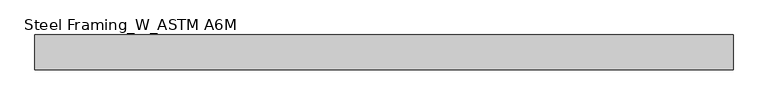
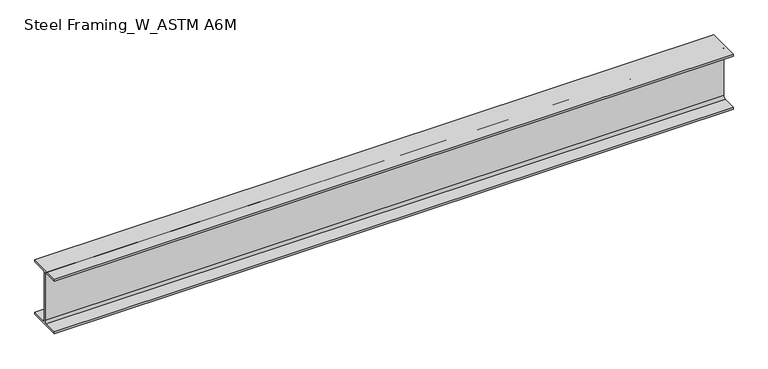
"""IFC4 building model written with IfcOpenShell, lengths in millimetres: beam geometry, Steel Framing_W_ASTM A6M : H_SB_ASB_W360x64."""

from ifc_helpers import new_model, si_unit, point, frame, frame_2d, origin, place, context, project, spatial, polyline, circle_curve, trimmed, segment, composite_curve, outline, extrude, source, transform, mapped, element, save


def steel_framing_w_astm_a6m_37d654f5(model_context):
    return source(origin(), model_context, "Body", "SweptSolid", [
        extrude(outline(composite_curve([segment(polyline([(101.5, -160.5), (101.5, -174.0), (-101.5, -174.0), (-101.5, -160.5), (-18.775, -160.5)]), True, "CONTINUOUS"), segment(trimmed(circle_curve(frame_2d((-18.775, -145.6)), 14.9), [point((-18.775, -160.5))], [point((-3.875, -145.6))], True, "CARTESIAN"), True, "CONTINUOUS"), segment(polyline([(-3.875, -145.6), (-3.875, 145.6)]), True, "CONTINUOUS"), segment(trimmed(circle_curve(frame_2d((-18.775, 145.6)), 14.9), [point((-3.875, 145.6))], [point((-18.775, 160.5))], True, "CARTESIAN"), True, "CONTINUOUS"), segment(polyline([(-18.775, 160.5), (-101.5, 160.5), (-101.5, 174.0), (101.5, 174.0), (101.5, 160.5), (18.775, 160.5)]), True, "CONTINUOUS"), segment(trimmed(circle_curve(frame_2d((18.775, 145.6)), 14.9), [point((18.775, 160.5))], [point((3.875, 145.6))], True, "CARTESIAN"), True, "CONTINUOUS"), segment(polyline([(3.875, 145.6), (3.875, -145.6)]), True, "CONTINUOUS"), segment(trimmed(circle_curve(frame_2d((18.775, -145.6)), 14.9), [point((3.875, -145.6))], [point((18.775, -160.5))], True, "CARTESIAN"), True, "CONTINUOUS"), segment(polyline([(18.775, -160.5), (101.5, -160.5)]), True, "CONTINUOUS")], self_intersect=False)), frame((-2037.3, 0.0, 0.0), z_axis=(1.0, 0.0, 0.0), x_axis=(0.0, 1.0, 0.0)), (0.0, 0.0, 1.0), 4074.6),
    ])


if __name__ == "__main__":
    model = new_model("IFC4")
    model_context = context("Model", 3, world=origin())
    ifc_project = project(units=[si_unit("LENGTHUNIT", "METRE", prefix="MILLI")], contexts=[model_context])
    site = spatial("IfcSite", under=ifc_project)
    building = spatial("IfcBuilding", under=site)
    placement = place(None, origin())
    steel_framing_w_astm_a6m_shape = steel_framing_w_astm_a6m_37d654f5(model_context)
    element("IfcBeam", 1, ObjectType="Steel Framing_W_ASTM A6M : H_SB_ASB_W360x64", at=placement, inside=building, context=model_context, shape_type="MappedRepresentation", body=[
        mapped(steel_framing_w_astm_a6m_shape, transform((0.0, 0.0, 0.0), x_axis=(1.0, 0.0, 0.0), y_axis=(0.0, 1.0, 0.0), z_axis=(0.0, 0.0, 1.0))),
    ])
    save(model, "model.ifc")

# Revit data of these elements
# Type "Steel Framing_W_ASTM A6M : H_SB_ASB_W360x64"
#   Section Name Key = "W14x43"
#   Width = 20.3 cm
#   Web Thickness = 0.775 cm
#   Web Fillet = 1.49 cm
#   Warping Constant = 524000.0 cm⁶
#   Torsional Moment of Inertia = 43.70 cm⁴
#   Section Area = 81.3 cm²
#   Plastic Modulus weak axis = 283.0 cm³
#   Plastic Modulus strong axis = 1140.0 cm³
#   Perimeter = 1.47 m²/m
#   Nominal Weight = 64.00 kgf/m
#   Moment of Inertia weak axis = 1880.00 cm⁴
#   Moment of Inertia strong axis = 17800.00 cm⁴
#   Height = 34.8 cm
#   Flange Thickness = 1.35 cm
#   Elastic Modulus weak axis = 185.0 cm³
#   Elastic Modulus strong axis = 1030.0 cm³
#   Centroid Vertical = 17.4 cm
#   Centroid Horizontal = 10.15 cm
#   Length [instance default] = 1500.000 mm
#   Structural Material [instance default] = Steel, 45-345
#   Bolt Spacing = 0
#   Assembly Code = ""
# Element 1 (IfcBeam, "Steel Framing_W_ASTM A6M : H_SB_ASB_W360x64")
#   Materials on its faces: "Steel, 45-345"
# Materials
#   "Steel, 45-345": class "Metal", colour RGB 189 187 185, transparency 0, Description = "Steel 345 MPa", Cost = 0
